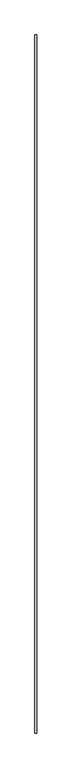
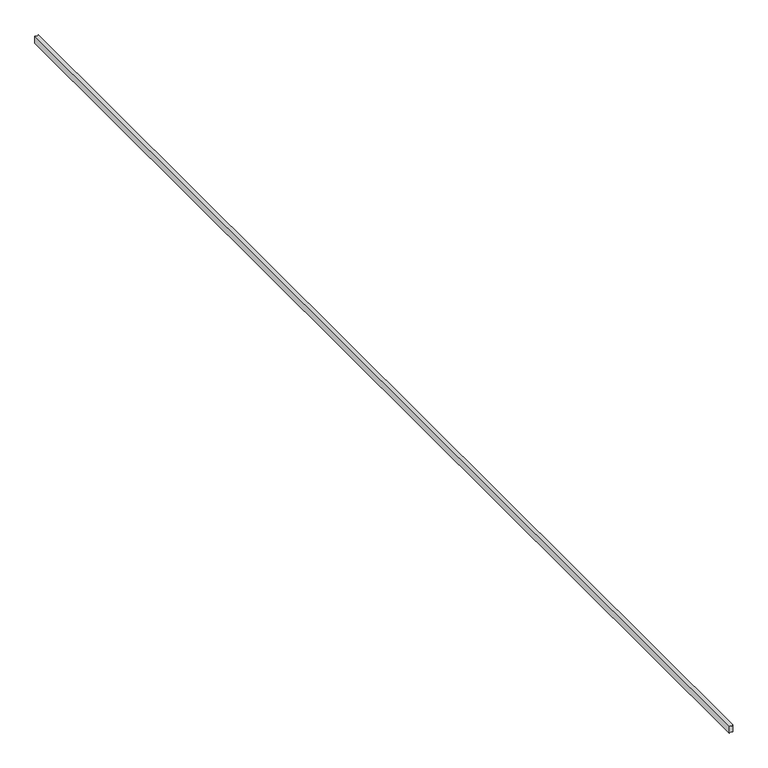
"""IFC4 building model written with IfcOpenShell, lengths in millimetres: proxy geometry, Joint044 17099 : Joint044 17099."""

from ifc_helpers import new_model, si_unit, point, frame, frame_2d, origin, place, context, project, spatial, polyline, circle_curve, trimmed, segment, composite_curve, outline, extrude, source, transform, mapped, element, save


def generic_models_9eafe6f1(model_context):
    return source(origin(), model_context, "Body", "SweptSolid", [
        extrude(outline(composite_curve([segment(polyline([(41291.6228899, 6044.4395748), (41303.9837728, 6044.4395748)]), True, "CONTINUOUS"), segment(trimmed(circle_curve(frame_2d((41306.6762213, 6041.4695305)), 4.0087956), [point((41303.9837728, 6044.4395748))], [point((41303.9837728, 6038.4994861))], True, "CARTESIAN"), True, "CONTINUOUS"), segment(polyline([(41303.9837728, 6038.4994861), (41291.6228899, 6038.4994861)]), True, "CONTINUOUS"), segment(trimmed(circle_curve(frame_2d((41289.5429789, 6041.4695305)), 3.6259059), [point((41291.6228899, 6038.4994861))], [point((41291.6228899, 6044.4395748))], True, "CARTESIAN"), True, "CONTINUOUS")], self_intersect=False)), frame((0.0, 2217.3609988, 0.0), z_axis=(0.0, 1.0, 0.0), x_axis=(0.0, 0.0, 1.0)), (0.0, 0.0, 1.0), 2000.0),
    ])


if __name__ == "__main__":
    model = new_model("IFC4")
    model_context = context("Model", 3, world=origin())
    ifc_project = project(units=[si_unit("LENGTHUNIT", "METRE", prefix="MILLI")], contexts=[model_context])
    site = spatial("IfcSite", under=ifc_project)
    building = spatial("IfcBuilding", under=site)
    placement = place(None, origin())
    generic_models_shape = generic_models_9eafe6f1(model_context)
    element("IfcBuildingElementProxy", 1, Name="Joint044 17099 : Joint044 17099", ObjectType="Joint044 17099 : Joint044 17099", at=placement, inside=building, context=model_context, shape_type="MappedRepresentation", body=[
        mapped(generic_models_shape, transform((0.0, 0.0, 0.0), x_axis=(1.0, 0.0, 0.0), y_axis=(0.0, 1.0, 0.0), z_axis=(0.0, 0.0, 1.0))),
    ])
    save(model, "model.ifc")

# Revit data of these elements
# Type "Joint044 17099 : Joint044 17099"
#   NameOverride = "Joint044"
# Element 1 (IfcBuildingElementProxy, "Joint044 17099 : Joint044 17099")
#   Materials on its faces: "SEALANT"
# Materials
#   "SEALANT": class "Unassigned", colour RGB 142 225 148, transparency 0
